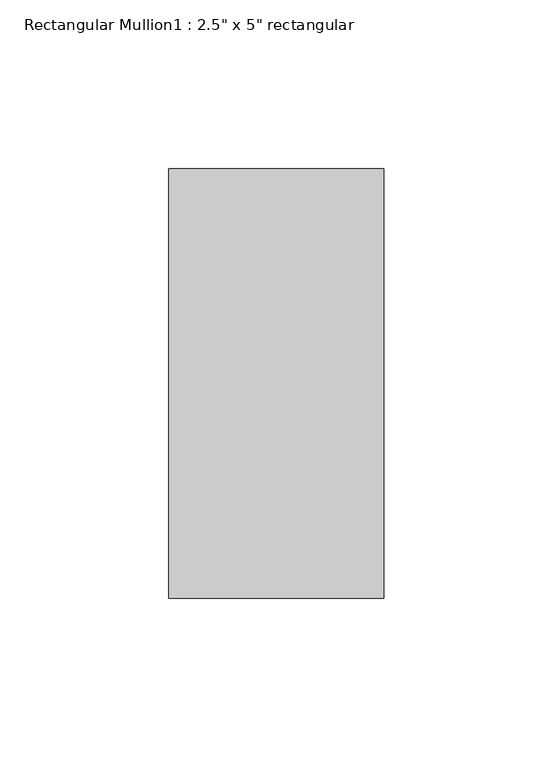
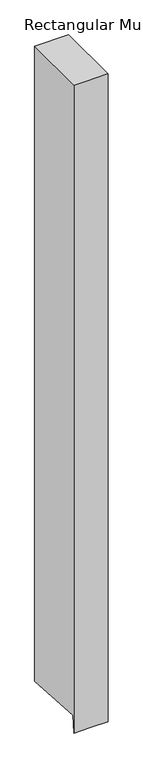
"""IFC4 building model written with IfcOpenShell, lengths in millimetres: member geometry."""

import ifcopenshell
import ifcopenshell.guid

model = None  # the IFC model being written
_history = None  # IfcOwnerHistory: only IFC2X3 demands one
_inside = {}  # id of a spatial element -> (the spatial element, [elements in it])
_under = {}  # id of a project, library or spatial element -> (it, [spatial elements below it])
_declared = {}  # id of a project -> (the project, [libraries it declares])
_typed = {}  # id of a type object -> (the type object, [elements of that type])
_made_of = {}  # id of a material, layer set ... -> (it, [elements and type objects made of it])


def new_model(schema):
    """Start an empty IFC model of exactly this schema.

    Asked for "IFC4X3", IfcOpenShell would pick the latest addendum, in which some entities
    have other attributes; the version numbers below select the first issue.
    IFC2X3 requires an IfcOwnerHistory on every rooted entity: one is made here for all.
    """
    global model, _history
    if schema == "IFC4X3":
        model = ifcopenshell.file(schema_version=(4, 3, 0, 0))
    else:
        model = ifcopenshell.file(schema=schema)
    _inside.clear()
    _under.clear()
    _declared.clear()
    _typed.clear()
    _made_of.clear()
    _history = None
    if model.schema == "IFC2X3":
        org = make("IfcOrganization", Name="unknown")
        user = make(
            "IfcPersonAndOrganization",
            ThePerson=make("IfcPerson", FamilyName="unknown"),
            TheOrganization=org,
        )
        app = make(
            "IfcApplication",
            ApplicationDeveloper=org,
            Version="unknown",
            ApplicationFullName="unknown",
            ApplicationIdentifier="unknown",
        )
        _history = make(
            "IfcOwnerHistory",
            OwningUser=user,
            OwningApplication=app,
            ChangeAction="ADDED",
            CreationDate=0,
        )
    return model


def make(cls, **values):
    """One entity of the class cls with the attributes given. An attribute that is None is left unset."""
    return model.create_entity(
        cls, **{name: value for name, value in values.items() if value is not None}
    )


def rooted(cls, **values):
    """An entity with a GlobalId (a new one), such as an element, a storey or a relation."""
    return make(cls, GlobalId=ifcopenshell.guid.new(), OwnerHistory=_history, **values)


def si_unit(unit_type, name, prefix=None):
    """IfcSIUnit, for example si_unit("LENGTHUNIT", "METRE", prefix="MILLI")."""
    return make("IfcSIUnit", UnitType=unit_type, Prefix=prefix, Name=name)


def assignment(units):
    """IfcUnitAssignment: the units of a project."""
    return None if units is None else make("IfcUnitAssignment", Units=units)


def point(xyz):
    """IfcCartesianPoint."""
    return None if xyz is None else make("IfcCartesianPoint", Coordinates=xyz)


def direction(xyz):
    """IfcDirection."""
    return None if xyz is None else make("IfcDirection", DirectionRatios=xyz)


def frame(location, z_axis=None, x_axis=None):
    """IfcAxis2Placement3D, a coordinate frame: its origin and axes. An axis left out is left unset."""
    return make(
        "IfcAxis2Placement3D",
        Location=point(location),
        Axis=direction(z_axis),
        RefDirection=direction(x_axis),
    )


def origin():
    """The frame at (0, 0, 0) with its axes left unset."""
    return frame((0.0, 0.0, 0.0))


def place(relative_to, where):
    """IfcLocalPlacement: puts the frame where relative to a parent placement (None: the world)."""
    return make(
        "IfcLocalPlacement", PlacementRelTo=relative_to, RelativePlacement=where
    )


def context(
    kind, dimensions, precision=None, world=None, true_north=None, identifier=None
):
    """IfcGeometricRepresentationContext, for example the 3D "Model" context."""
    return make(
        "IfcGeometricRepresentationContext",
        ContextIdentifier=identifier,
        ContextType=kind,
        CoordinateSpaceDimension=dimensions,
        Precision=precision,
        WorldCoordinateSystem=world,
        TrueNorth=true_north,
    )


def project(units=None, contexts=None):
    """IfcProject with its units and contexts."""
    return rooted(
        "IfcProject",
        Name="project",
        RepresentationContexts=contexts,
        UnitsInContext=assignment(units),
    )


def spatial(cls, under=None, at=None, **own):
    """A site, building, storey or space (cls), placed at a placement, below another one or the project."""
    s = rooted(cls, ObjectPlacement=at, **own)
    if under is not None:
        _under.setdefault(under.id(), (under, []))[1].append(s)
    return s


def faces_of(points, faces, orient=None, outer=None):
    """IfcFace entities. A face is a list of loops; a loop is a list of indices into points, from 0.

    orient and outer hold one flag for each loop. By default every Orientation is true, the
    first loop of a face is its IfcFaceOuterBound and the others are IfcFaceBound.
    """
    made = []
    for i, loops in enumerate(faces):
        bounds = []
        for j, loop in enumerate(loops):
            is_outer = j == 0 if outer is None else outer[i][j]
            bounds.append(
                make(
                    "IfcFaceOuterBound" if is_outer else "IfcFaceBound",
                    Bound=make("IfcPolyLoop", Polygon=[points[k] for k in loop]),
                    Orientation=True if orient is None else orient[i][j],
                )
            )
        made.append(make("IfcFace", Bounds=bounds))
    return made


def faceted_brep(points, faces, orient=None, outer=None, voids=None):
    """IfcFacetedBrep: a solid bounded by flat faces; with voids (closed shells), ...WithVoids."""
    shared = [point(p) for p in points]
    hull = make("IfcClosedShell", CfsFaces=faces_of(shared, faces, orient, outer))
    if voids is None:
        return make("IfcFacetedBrep", Outer=hull)
    return make(
        "IfcFacetedBrepWithVoids",
        Outer=hull,
        Voids=[
            make(cls, CfsFaces=faces_of(shared, fs, o, b)) for cls, fs, o, b in voids
        ],
    )


def shape(context_of_items, identifier, shape_type, items):
    """IfcShapeRepresentation: the items that make up one representation, for example the "Body"."""
    return make(
        "IfcShapeRepresentation",
        ContextOfItems=context_of_items,
        RepresentationIdentifier=identifier,
        RepresentationType=shape_type,
        Items=items,
    )


def source(mapping_origin, context_of_items, identifier, shape_type, items):
    """IfcRepresentationMap: a shape defined once, which mapped items show again and again."""
    return make(
        "IfcRepresentationMap",
        MappingOrigin=mapping_origin,
        MappedRepresentation=shape(context_of_items, identifier, shape_type, items),
    )


def transform(
    local_origin,
    x_axis=None,
    y_axis=None,
    z_axis=None,
    scale=None,
    scale2=None,
    scale3=None,
    uniform=True,
):
    """IfcCartesianTransformationOperator3D, or its non-uniform kind. x_axis, y_axis, z_axis: its Axis1, 2, 3."""
    if uniform:
        return make(
            "IfcCartesianTransformationOperator3D",
            Axis1=direction(x_axis),
            Axis2=direction(y_axis),
            LocalOrigin=point(local_origin),
            Scale=scale,
            Axis3=direction(z_axis),
        )
    return make(
        "IfcCartesianTransformationOperator3DnonUniform",
        Axis1=direction(x_axis),
        Axis2=direction(y_axis),
        LocalOrigin=point(local_origin),
        Scale=scale,
        Axis3=direction(z_axis),
        Scale2=scale2,
        Scale3=scale3,
    )


def mapped(mapping_source, mapping_target):
    """IfcMappedItem: shows the shape of a source again, moved by a transform."""
    return make(
        "IfcMappedItem", MappingSource=mapping_source, MappingTarget=mapping_target
    )


def made_of(thing, what):
    """Note that an element or type object is made of a material, layer set ...; save() writes the relation."""
    if what is not None:
        _made_of.setdefault(what.id(), (what, []))[1].append(thing)
    return thing


def element(
    cls,
    number,
    at=None,
    inside=None,
    cuts=None,
    type_object=None,
    material=None,
    context=None,
    identifier="Body",
    shape_type=None,
    held_by="IfcProductDefinitionShape",
    body=None,
    shapes=None,
    **own,
):
    """One element of the class cls, such as IfcWall. Its Tag is "e" and its number.

    at: its placement. inside: the storey or other place that contains it. cuts: it is an
    opening in that element (IfcRelVoidsElement). A single representation is given by context,
    identifier, shape_type and body (its items); several are given by shapes. held_by: the class
    of the entity that holds the representations. save() writes the other relations.
    """
    e = rooted(cls, Tag="e%d" % number, ObjectPlacement=at, **own)
    if body is not None:
        shapes = [shape(context, identifier, shape_type, body)]
    if shapes is not None:
        e.Representation = make(held_by, Representations=shapes)
    if inside is not None:
        _inside.setdefault(inside.id(), (inside, []))[1].append(e)
    if cuts is not None:
        rooted(
            "IfcRelVoidsElement", RelatingBuildingElement=cuts, RelatedOpeningElement=e
        )
    if type_object is not None:
        _typed.setdefault(type_object.id(), (type_object, []))[1].append(e)
    return made_of(e, material)


def aggregate(whole, parts):
    """IfcRelAggregates: a whole, such as a stair, and the parts it consists of."""
    return rooted("IfcRelAggregates", RelatingObject=whole, RelatedObjects=parts)


def save(model, path):
    """Write the relations noted so far, then the file.

    IfcRelAggregates (storeys below a building ...), IfcRelContainedInSpatialStructure (elements
    in a storey), IfcRelDefinesByType, IfcRelAssociatesMaterial and IfcRelDeclares: one each for
    every whole, place, type object, material and project.
    """
    for whole, parts in _under.values():
        aggregate(whole, parts)
    for where, things in _inside.values():
        rooted(
            "IfcRelContainedInSpatialStructure",
            RelatedElements=things,
            RelatingStructure=where,
        )
    for kind, things in _typed.values():
        rooted("IfcRelDefinesByType", RelatedObjects=things, RelatingType=kind)
    for what, things in _made_of.values():
        rooted("IfcRelAssociatesMaterial", RelatedObjects=things, RelatingMaterial=what)
    for by, libraries in _declared.values():
        rooted("IfcRelDeclares", RelatingContext=by, RelatedDefinitions=libraries)
    model.write(path)


def member_21287d99(model_context):
    return source(origin(), model_context, "Body", "Brep", [
        faceted_brep([(31.75, 63.5, 0.0), (-31.75, 63.5, 0.0), (-31.75, -63.5, 0.0), (31.75, -63.5, 0.0), (31.75, 63.5, -1253.5867756), (0.0, 63.5, -1253.5867756), (-31.75, 63.5, -1253.5867756), (-31.75, -61.1522336, -1244.9455147), (-31.75, -63.5, -1278.8126009), (0.0, -63.5, -1278.8126009), (31.75, -63.5, -1278.8126009), (31.75, -61.1522336, -1244.9455147), (0.0, -61.1522336, -1244.9455147)], [[[0, 1, 2, 3]], [[1, 0, 4, 5, 6]], [[2, 1, 6, 7, 8]], [[3, 2, 8, 9, 10]], [[0, 3, 10, 11, 4]], [[4, 11, 12, 5]], [[11, 10, 9, 12]], [[9, 8, 7, 12]], [[7, 6, 5, 12]]]),
    ])


if __name__ == "__main__":
    model = new_model("IFC4")
    model_context = context("Model", 3, world=origin())
    ifc_project = project(units=[si_unit("LENGTHUNIT", "METRE", prefix="MILLI")], contexts=[model_context])
    site = spatial("IfcSite", under=ifc_project)
    building = spatial("IfcBuilding", under=site)
    placement = place(None, origin())
    member_shape = member_21287d99(model_context)
    element("IfcMember", 1, ObjectType="Rectangular Mullion1 : 2.5\" x 5\" rectangular", at=placement, inside=building, context=model_context, shape_type="MappedRepresentation", body=[
        mapped(member_shape, transform((0.0, 0.0, 0.0), x_axis=(1.0, 0.0, 0.0), y_axis=(0.0, 1.0, 0.0), z_axis=(0.0, 0.0, 1.0))),
    ])
    save(model, "model.ifc")

# Revit data of these elements
# Type "Rectangular Mullion1 : 2.5\" x 5\" rectangular"
#   built-in parameter 1007304 = 0.416667 (stored number, unit not read)
#   built-in parameter 1007301 = 0.104167 (stored number, unit not read)
#   built-in parameter 1007300 = 0.104167 (stored number, unit not read)
# Element 1 (IfcMember, "Rectangular Mullion1 : 2.5\" x 5\" rectangular")
#   Materials on its faces: "support-frame"
# Materials
#   "support-frame": class "Unassigned", colour RGB 233 233 233, transparency 0, Cost = 0
